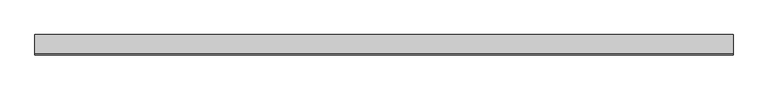
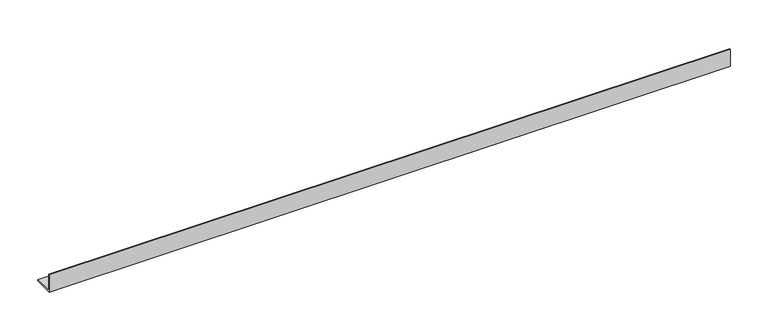
"""IFC4 building model written with IfcOpenShell, lengths in millimetres: proxy geometry, Generic Models 7:Generic Models 1:7:Generic Models 1:7 : Generic Models 7:Generic Models 1:337419:9 : Generic Models 7:Generic Models 1:7:Generic Models 1:7 : Generic Models 7:Generic Models 1:337419:315055."""

from ifc_helpers import new_model, si_unit, frame, origin, place, context, project, spatial, polyline, outline, extrude, source, transform, mapped, element, save


def generic_models_df988646(model_context):
    return source(origin(), model_context, "Body", "SweptSolid", [
        extrude(outline(polyline([(-579033.9952859, 46.8525192), (-579064.7942981, 46.8525192), (-579064.7942981, 74.9835291), (-579063.2067981, 74.9835291), (-579063.2067981, 48.4400192), (-579033.9952859, 48.4400192), (-579033.9952859, 46.8525192)])), frame((591714.0570845, 0.0, 0.0), z_axis=(1.0, 0.0, 0.0), x_axis=(0.0, 1.0, 0.0)), (0.0, 0.0, 1.0), 1044.8567691),
    ])


if __name__ == "__main__":
    model = new_model("IFC4")
    model_context = context("Model", 3, world=origin())
    ifc_project = project(units=[si_unit("LENGTHUNIT", "METRE", prefix="MILLI")], contexts=[model_context])
    site = spatial("IfcSite", under=ifc_project)
    building = spatial("IfcBuilding", under=site)
    placement = place(None, origin())
    generic_models_shape = generic_models_df988646(model_context)
    element("IfcBuildingElementProxy", 1, Name="Generic Models 7:Generic Models 1:7:Generic Models 1:7 : Generic Models 7:Generic Models 1:337419:9 : Generic Models 7:Generic Models 1:7:Generic Models 1:7 : Generic Models 7:Generic Models 1:337419:315055", ObjectType="Generic Models 7:Generic Models 1:7:Generic Models 1:7 : Generic Models 7:Generic Models 1:337419:9 : Generic Models 7:Generic Models 1:7:Generic Models 1:7 : Generic Models 7:Generic Models 1:337419:315055", at=placement, inside=building, context=model_context, shape_type="MappedRepresentation", body=[
        mapped(generic_models_shape, transform((0.0, 0.0, 0.0), x_axis=(1.0, 0.0, 0.0), y_axis=(0.0, 1.0, 0.0), z_axis=(0.0, 0.0, 1.0))),
    ])
    save(model, "model.ifc")

# Revit data of these elements
# Type "Generic Models 7:Generic Models 1:7:Generic Models 1:7 : Generic Models 7:Generic Models 1:337419:9 : Generic Models 7:Generic Models 1:7:Generic Models 1:7 : Generic Models 7:Generic Models 1:337419:315055"
#   NameOverride = "Generic Models 7:Generic Models 1:7:Generic Models 1:7 : Generic Models 7:Generic Models 1:337419:315055"
#   ObjectTypeOverride = "Generic Models 1:7 : Generic Models 7:Generic Models 1:337419"
#   Reference = "Generic Models 1"
#   Tag = "315055"
# Element 1 (IfcBuildingElementProxy, "Generic Models 7:Generic Models 1:7:Generic Models 1:7 : Generic Models 7:Generic Models 1:337419:9 : Generic Models 7:Generic Models 1:7:Generic Models 1:7 : Generic Models 7:Generic Models 1:337419:315055")
#   Materials on its faces: "STAINLESS STEEL BENT PLATE (FLASHING)"
# Materials
#   "STAINLESS STEEL BENT PLATE (FLASHING)": class "Unassigned", colour RGB 210 209 208, transparency 0, Cost = 0
